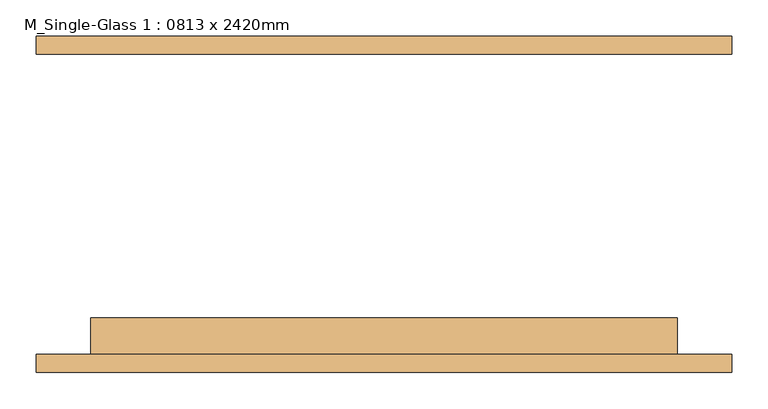
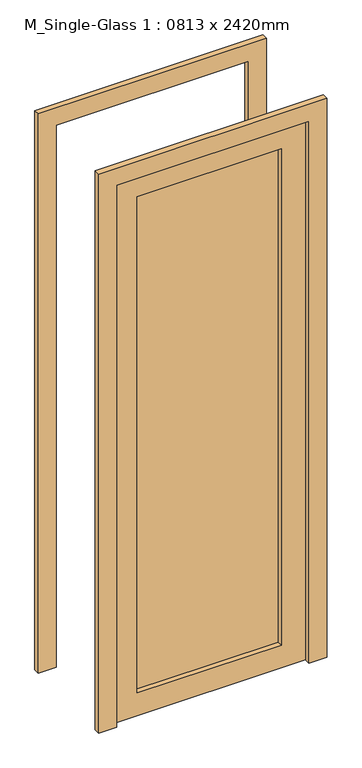
"""IFC4 building model written with IfcOpenShell, lengths in millimetres: door geometry, M_Single-Glass 1 : 0813 x 2420mm."""

from ifc_helpers import new_model, si_unit, frame, origin, place, context, project, spatial, polyline, outline, extrude, source, transform, mapped, element, save


def m_single_glass_1_0813_x_2420mm_c90ba5ca(model_context):
    return source(origin(), model_context, "Body", "SweptSolid", [
        extrude(outline(polyline([(2420.0, 406.5), (0.0, 406.5), (0.0, 482.5), (2496.0, 482.5), (2496.0, -482.5), (0.0, -482.5), (0.0, -406.5), (2420.0, -406.5), (2420.0, 406.5)])), frame((0.0, 208.5, 0.0), z_axis=(0.0, 1.0, 0.0), x_axis=(0.0, 0.0, 1.0)), (0.0, 0.0, 1.0), 25.0),
        extrude(outline(polyline([(2420.0, 406.5), (0.0, 406.5), (0.0, 482.5), (2496.0, 482.5), (2496.0, -482.5), (0.0, -482.5), (0.0, -406.5), (2420.0, -406.5), (2420.0, 406.5)])), frame((0.0, -233.5, 0.0), z_axis=(0.0, 1.0, 0.0), x_axis=(0.0, 0.0, 1.0)), (0.0, 0.0, 1.0), 25.0),
        extrude(outline(polyline([(304.5, -179.925), (304.5, -186.275), (-304.5, -186.275), (-304.5, -179.925), (304.5, -179.925)])), frame((0.0, 0.0, 102.0), z_axis=(0.0, 0.0, 1.0), x_axis=(1.0, 0.0, 0.0)), (0.0, 0.0, 1.0), 2216.0),
        extrude(outline(polyline([(2420.0, 406.5), (2420.0, -406.5), (0.0, -406.5), (0.0, 406.5), (2420.0, 406.5)]), holes=[polyline([(2318.0, -304.5), (2318.0, 304.5), (102.0, 304.5), (102.0, -304.5), (2318.0, -304.5)])]), frame((0.0, -208.5, 0.0), z_axis=(0.0, 1.0, 0.0), x_axis=(0.0, 0.0, 1.0)), (0.0, 0.0, 1.0), 51.0),
    ])


if __name__ == "__main__":
    model = new_model("IFC4")
    model_context = context("Model", 3, world=origin())
    ifc_project = project(units=[si_unit("LENGTHUNIT", "METRE", prefix="MILLI")], contexts=[model_context])
    site = spatial("IfcSite", under=ifc_project)
    building = spatial("IfcBuilding", under=site)
    placement = place(None, origin())
    m_single_glass_1_0813_x_2420mm_shape = m_single_glass_1_0813_x_2420mm_c90ba5ca(model_context)
    element("IfcDoor", 1, ObjectType="M_Single-Glass 1 : 0813 x 2420mm", at=placement, inside=building, context=model_context, shape_type="MappedRepresentation", body=[
        mapped(m_single_glass_1_0813_x_2420mm_shape, transform((0.0, 0.0, 0.0), x_axis=(1.0, 0.0, 0.0), y_axis=(0.0, 1.0, 0.0), z_axis=(0.0, 0.0, 1.0))),
    ])
    save(model, "model.ifc")

# Revit data of these elements
# Type "M_Single-Glass 1 : 0813 x 2420mm"
#   Manufacturer = "Manufacturer"
#   Type Mark = "56"
#   Construction Type = "Construction Type"
#   Fire Rating = "Fire Rating"
#   AccessibilityPerformance = "AccessibilityPerformance"
#   CodePerformance = "CodePerformance"
#   IsFireExit = "IsFireExit"
#   ConstructionType = "ConstructionType"
#   GlazingAreaFraction = "GlazingAreaFraction"
#   OperationType = "OperationType"
#   Area = "Area"
#   Color = "Color"
#   Constituents = "Constituents"
#   Features = "Features"
#   Finish = "Finish"
#   Grade = "Grade"
#   Material = "Material"
#   ModelReference = "ModelReference"
#   NominalHeight = "NominalHeight"
#   NominalLength = "NominalLength"
#   NominalWidth = "NominalWidth"
#   ProductionYear = "ProductionYear"
#   Reference = "Reference"
#   Shape = "Shape"
#   Size = "Size"
#   SustainabilityPerformance = "SustainabilityPerformance"
#   WarrantyDescription = "WarrantyDescription"
#   WarrantyDurationLabor = "WarrantyDurationLabor"
#   WarrantyDurationParts = "WarrantyDurationParts"
#   WarrantyGuarantorLabor = "WarrantyGuarantorLabor"
#   WarrantyGuarantorParts = "WarrantyGuarantorParts"
#   ExpectedLife = "ExpectedLife"
#   ReplacementCost = "ReplacementCost"
#   AssetAccountingType = "FIXED"
#   ModelLabel = "ModelLabel"
#   Thickness = 0.051 m
#   Height = 2.420 m
#   Rail Width - Base = 0.102 m
#   Rail Width - Top = 0.102 m
#   Stile Width - Hinge = 0.102 m
#   Stile Width - Latch = 0.102 m
#   Trim Projection Ext = 0.025 m
#   Trim Projection Int = 0.025 m
#   Trim Width = 0.076 m
#   Width = 0.813 m
#   Function = 1
#   Door Material = Door - Panel
#   Frame Material = Door - Frame
#   Wall Closure = (empty or 0)
# Element 1 (IfcDoor, "M_Single-Glass 1 : 0813 x 2420mm")
#   Materials on its faces: "Door - Frame", "Door - Panel", "Glass"
# Materials
#   "Door - Panel": class "Wood", colour RGB 210 159 95, transparency 0
#   "Door - Frame": class "Miscellaneous", colour RGB 118 70 51, transparency 0
#   "Glass": class "Glass", colour RGB 0 128 192, transparency 0.9
